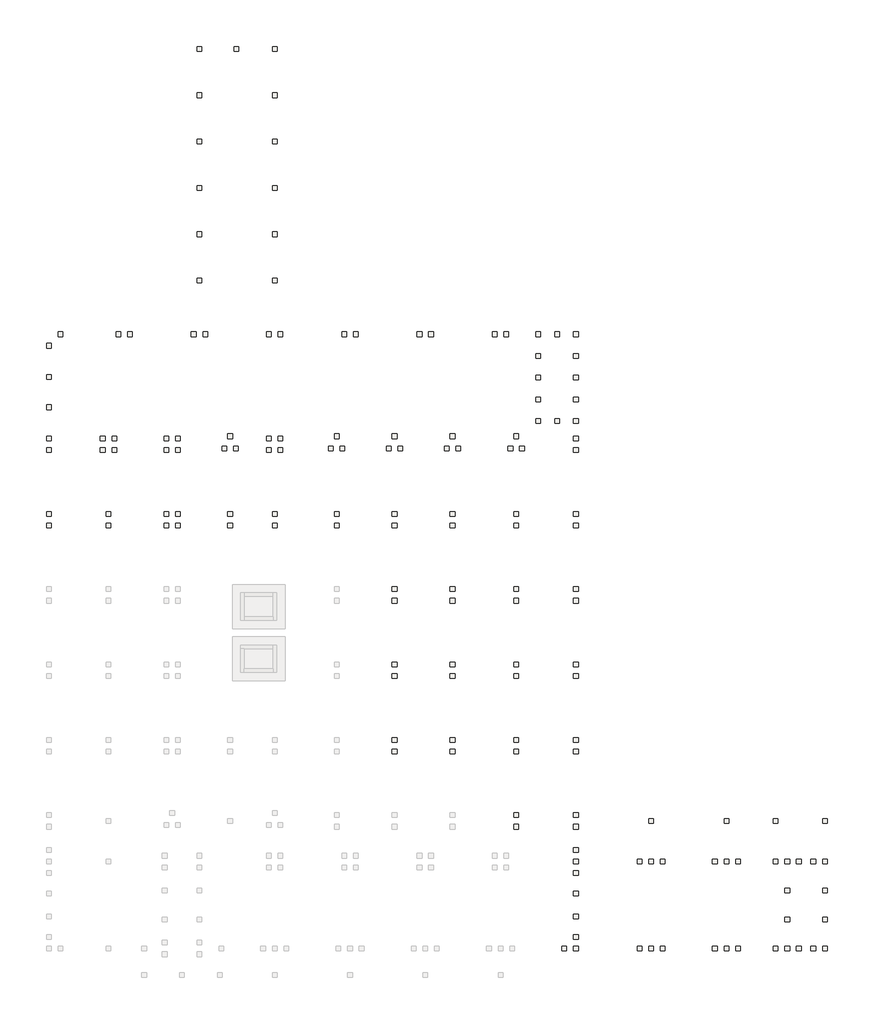
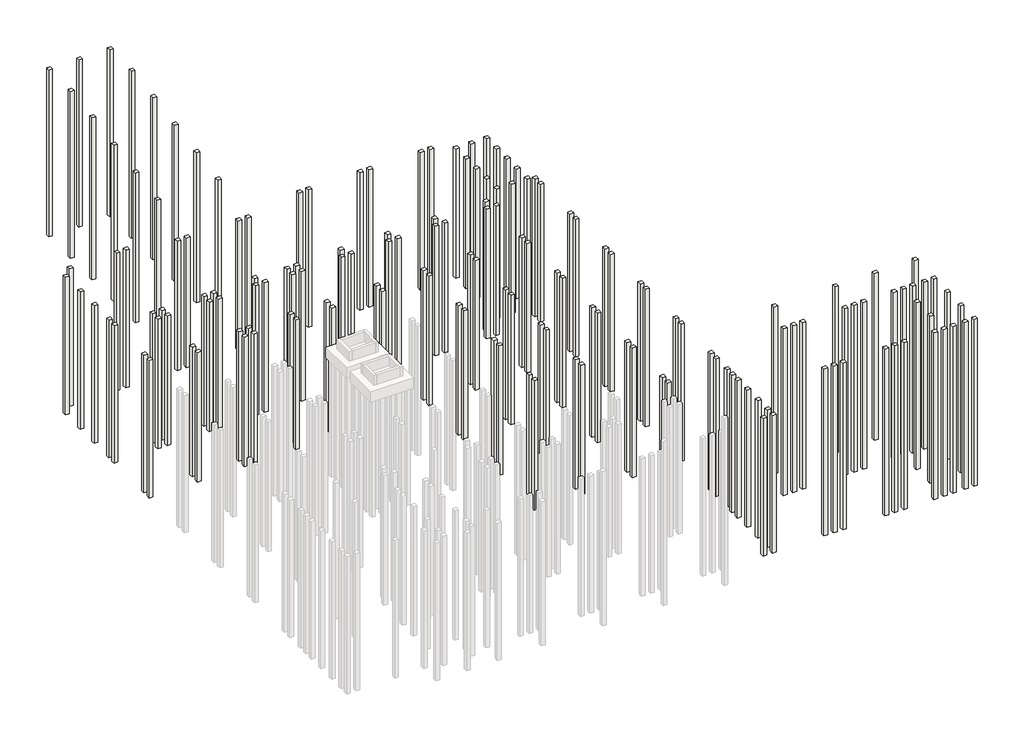
# Not in any storey, part 2 of 2: 160 footings.
# Revit data of these elements (continued)
# Element 105 (IfcFooting, "NLRS_17_SFO_TLB_funderingspaal geheid beton prefab-AV-MMBPC_gen_rsf : heipaal beton prefab_gen__bxh 400x400") (continued)
#   NLRS_S_draagvermogen_druk = 0.00 kN
#   Angle = 0.00°
#   IsExternal = yes
#   LoadBearing = yes
#   Slanted = 0
#   Phase Created = NLRS_nieuw
#   Materials on its faces: "NLRS_f2_beton prefab_gen_rsf"
# Element 106 (IfcFooting, "NLRS_17_SFO_TLB_funderingspaal geheid beton prefab-AV-MMBPC_gen_rsf : heipaal beton prefab_gen__bxh 400x400")
#   IfcGUID = "3loy75XKz2Rw4dS8JWiatC"
#   Slanted Angle = 0.00°
#   NLRS_S_draagvermogen_trek = 0.00 kN
#   NLRS_S_draagvermogen_druk = 0.00 kN
#   Angle = 0.00°
#   IsExternal = yes
#   LoadBearing = yes
#   Slanted = 0
#   Phase Created = NLRS_nieuw
#   Materials on its faces: "NLRS_f2_beton prefab_gen_rsf"
# Element 107 (IfcFooting, "NLRS_17_SFO_TLB_funderingspaal geheid beton prefab-AV-MMBPC_gen_rsf : heipaal beton prefab_gen__bxh 400x400")
#   IfcGUID = "3loy75XKz2Rw4dS8JWiatv"
#   Slanted Angle = 0.00°
#   NLRS_S_draagvermogen_trek = 0.00 kN
#   NLRS_S_draagvermogen_druk = 0.00 kN
#   Angle = 0.00°
#   IsExternal = yes
#   LoadBearing = yes
#   Slanted = 0
#   Phase Created = NLRS_nieuw
#   Materials on its faces: "NLRS_f2_beton prefab_gen_rsf"
# Element 108 (IfcFooting, "NLRS_17_SFO_TLB_funderingspaal geheid beton prefab-AV-MMBPC_gen_rsf : heipaal beton prefab_gen__bxh 400x400")
#   IfcGUID = "3loy75XKz2Rw4dS8JWiat$"
#   Slanted Angle = 0.00°
#   NLRS_S_draagvermogen_trek = 0.00 kN
#   NLRS_S_draagvermogen_druk = 0.00 kN
#   Angle = 0.00°
#   IsExternal = yes
#   LoadBearing = yes
#   Slanted = 0
#   Phase Created = NLRS_nieuw
#   Materials on its faces: "NLRS_f2_beton prefab_gen_rsf"
# Element 109 (IfcFooting, "NLRS_17_SFO_TLB_funderingspaal geheid beton prefab-AV-MMBPC_gen_rsf : heipaal beton prefab_gen__bxh 400x400")
#   IfcGUID = "3loy75XKz2Rw4dS8JWiaEQ"
#   Slanted Angle = 0.00°
#   NLRS_S_draagvermogen_trek = 0.00 kN
#   NLRS_S_draagvermogen_druk = 0.00 kN
#   Angle = 0.00°
#   IsExternal = yes
#   LoadBearing = yes
#   Slanted = 0
#   Phase Created = NLRS_nieuw
#   Materials on its faces: "NLRS_f2_beton prefab_gen_rsf"
# Element 110 (IfcFooting, "NLRS_17_SFO_TLB_funderingspaal geheid beton prefab-AV-MMBPC_gen_rsf : heipaal beton prefab_gen__bxh 400x400")
#   IfcGUID = "3loy75XKz2Rw4dS8JWiaEW"
#   Slanted Angle = 0.00°
#   NLRS_S_draagvermogen_trek = 0.00 kN
#   NLRS_S_draagvermogen_druk = 0.00 kN
#   Angle = 0.00°
#   IsExternal = yes
#   LoadBearing = yes
#   Slanted = 0
#   Phase Created = NLRS_nieuw
#   Materials on its faces: "NLRS_f2_beton prefab_gen_rsf"
# Element 111 (IfcFooting, "NLRS_17_SFO_TLB_funderingspaal geheid beton prefab-AV-MMBPC_gen_rsf : heipaal beton prefab_gen__bxh 400x400")
#   IfcGUID = "3loy75XKz2Rw4dS8JWia10"
#   Slanted Angle = 0.00°
#   NLRS_S_draagvermogen_trek = 0.00 kN
#   NLRS_S_draagvermogen_druk = 0.00 kN
#   Angle = 0.00°
#   IsExternal = yes
#   LoadBearing = yes
#   Slanted = 0
#   Phase Created = NLRS_nieuw
#   Materials on its faces: "NLRS_f2_beton prefab_gen_rsf"
# Element 112 (IfcFooting, "NLRS_17_SFO_TLB_funderingspaal geheid beton prefab-AV-MMBPC_gen_rsf : heipaal beton prefab_gen__bxh 400x400")
#   IfcGUID = "3loy75XKz2Rw4dS8JWia16"
#   Slanted Angle = 0.00°
#   NLRS_S_draagvermogen_trek = 0.00 kN
#   NLRS_S_draagvermogen_druk = 0.00 kN
#   Angle = 0.00°
#   IsExternal = yes
#   LoadBearing = yes
#   Slanted = 0
#   Phase Created = NLRS_nieuw
#   Materials on its faces: "NLRS_f2_beton prefab_gen_rsf"
# Element 113 (IfcFooting, "NLRS_17_SFO_TLB_funderingspaal geheid beton prefab-AV-MMBPC_gen_rsf : heipaal beton prefab_gen__bxh 400x400")
#   IfcGUID = "3loy75XKz2Rw4dS8JWia1p"
#   Slanted Angle = 0.00°
#   NLRS_S_draagvermogen_trek = 0.00 kN
#   NLRS_S_draagvermogen_druk = 0.00 kN
#   Angle = 0.00°
#   IsExternal = yes
#   LoadBearing = yes
#   Slanted = 0
#   Phase Created = NLRS_nieuw
#   Materials on its faces: "NLRS_f2_beton prefab_gen_rsf"
# Element 114 (IfcFooting, "NLRS_17_SFO_TLB_funderingspaal geheid beton prefab-AV-MMBPC_gen_rsf : heipaal beton prefab_gen__bxh 400x400")
#   IfcGUID = "3loy75XKz2Rw4dS8JWia1n"
#   Slanted Angle = 0.00°
#   NLRS_S_draagvermogen_trek = 0.00 kN
#   NLRS_S_draagvermogen_druk = 0.00 kN
#   Angle = 0.00°
#   IsExternal = yes
#   LoadBearing = yes
#   Slanted = 0
#   Phase Created = NLRS_nieuw
#   Materials on its faces: "NLRS_f2_beton prefab_gen_rsf"
# Element 115 (IfcFooting, "NLRS_17_SFO_TLB_funderingspaal geheid beton prefab-AV-MMBPC_gen_rsf : heipaal beton prefab_gen__bxh 400x400")
#   IfcGUID = "3loy75XKz2Rw4dS8JWia5x"
#   Slanted Angle = 0.00°
#   NLRS_S_draagvermogen_trek = 0.00 kN
#   NLRS_S_draagvermogen_druk = 0.00 kN
#   Angle = 0.00°
#   IsExternal = yes
#   LoadBearing = yes
#   Slanted = 0
#   Phase Created = NLRS_nieuw
#   Materials on its faces: "NLRS_f2_beton prefab_gen_rsf"
# Element 116 (IfcFooting, "NLRS_17_SFO_TLB_funderingspaal geheid beton prefab-AV-MMBPC_gen_rsf : heipaal beton prefab_gen__bxh 400x400")
#   IfcGUID = "3loy75XKz2Rw4dS8JWia4Y"
#   Slanted Angle = 0.00°
#   NLRS_S_draagvermogen_trek = 0.00 kN
#   NLRS_S_draagvermogen_druk = 0.00 kN
#   Angle = 0.00°
#   IsExternal = yes
#   LoadBearing = yes
#   Slanted = 0
#   Phase Created = NLRS_nieuw
#   Materials on its faces: "NLRS_f2_beton prefab_gen_rsf"
# Element 117 (IfcFooting, "NLRS_17_SFO_TLB_funderingspaal geheid beton prefab-AV-MMBPC_gen_rsf : heipaal beton prefab_gen__bxh 400x400")
#   IfcGUID = "3loy75XKz2Rw4dS8JWia4W"
#   Slanted Angle = 0.00°
#   NLRS_S_draagvermogen_trek = 0.00 kN
#   NLRS_S_draagvermogen_druk = 0.00 kN
#   Angle = 0.00°
#   IsExternal = yes
#   LoadBearing = yes
#   Slanted = 0
#   Phase Created = NLRS_nieuw
#   Materials on its faces: "NLRS_f2_beton prefab_gen_rsf"
# Element 118 (IfcFooting, "NLRS_17_SFO_TLB_funderingspaal geheid beton prefab-AV-MMBPC_gen_rsf : heipaal beton prefab_gen__bxh 400x400")
#   IfcGUID = "1JrsWFyZX6xPuD52juGVxa"
#   Slanted Angle = 0.00°
#   NLRS_S_draagvermogen_trek = 0.00 kN
#   NLRS_S_draagvermogen_druk = 0.00 kN
#   Angle = 0.00°
#   IsExternal = yes
#   LoadBearing = yes
#   Slanted = 0
#   Phase Created = NLRS_nieuw
#   Materials on its faces: "NLRS_f2_beton prefab_gen_rsf"
# Element 119 (IfcFooting, "NLRS_17_SFO_TLB_funderingspaal geheid beton prefab-AV-MMBPC_gen_rsf : heipaal beton prefab_gen__bxh 400x400")
#   IfcGUID = "1JrsWFyZX6xPuD52juGVvn"
#   Slanted Angle = 0.00°
#   NLRS_S_draagvermogen_trek = 0.00 kN
#   NLRS_S_draagvermogen_druk = 0.00 kN
#   Angle = 0.00°
#   IsExternal = yes
#   LoadBearing = yes
#   Slanted = 0
#   Phase Created = NLRS_nieuw
#   Materials on its faces: "NLRS_f2_beton prefab_gen_rsf"
# Element 120 (IfcFooting, "NLRS_17_SFO_TLB_funderingspaal geheid beton prefab-AV-MMBPC_gen_rsf : heipaal beton prefab_gen__bxh 400x400")
#   IfcGUID = "1JrsWFyZX6xPuD52juGVv2"
#   Slanted Angle = 0.00°
#   NLRS_S_draagvermogen_trek = 0.00 kN
#   NLRS_S_draagvermogen_druk = 0.00 kN
#   Angle = 0.00°
#   IsExternal = yes
#   LoadBearing = yes
#   Slanted = 0
#   Phase Created = NLRS_nieuw
#   Materials on its faces: "NLRS_f2_beton prefab_gen_rsf"
# Element 121 (IfcFooting, "NLRS_17_SFO_TLB_funderingspaal geheid beton prefab-AV-MMBPC_gen_rsf : heipaal beton prefab_gen__bxh 400x400")
#   IfcGUID = "1JrsWFyZX6xPuD52juGV_f"
#   Slanted Angle = 0.00°
#   NLRS_S_draagvermogen_trek = 0.00 kN
#   NLRS_S_draagvermogen_druk = 0.00 kN
#   Angle = 0.00°
#   IsExternal = yes
#   LoadBearing = yes
#   Slanted = 0
#   Phase Created = NLRS_nieuw
#   Materials on its faces: "NLRS_f2_beton prefab_gen_rsf"
# Element 122 (IfcFooting, "NLRS_17_SFO_TLB_funderingspaal geheid beton prefab-AV-MMBPC_gen_rsf : heipaal beton prefab_gen__bxh 400x400")
#   IfcGUID = "1JrsWFyZX6xPuD52juGV_d"
#   Slanted Angle = 0.00°
#   NLRS_S_draagvermogen_trek = 0.00 kN
#   NLRS_S_draagvermogen_druk = 0.00 kN
#   Angle = 0.00°
#   IsExternal = yes
#   LoadBearing = yes
#   Slanted = 0
#   Phase Created = NLRS_nieuw
#   Materials on its faces: "NLRS_f2_beton prefab_gen_rsf"
# Element 123 (IfcFooting, "NLRS_17_SFO_TLB_funderingspaal geheid beton prefab-AV-MMBPC_gen_rsf : heipaal beton prefab_gen__bxh 400x400")
#   IfcGUID = "1JrsWFyZX6xPuD52juGV_b"
#   Slanted Angle = 0.00°
#   NLRS_S_draagvermogen_trek = 0.00 kN
#   NLRS_S_draagvermogen_druk = 0.00 kN
#   Angle = 0.00°
#   IsExternal = yes
#   LoadBearing = yes
#   Slanted = 0
#   Phase Created = NLRS_nieuw
#   Materials on its faces: "NLRS_f2_beton prefab_gen_rsf"
# Element 124 (IfcFooting, "NLRS_17_SFO_TLB_funderingspaal geheid beton prefab-AV-MMBPC_gen_rsf : heipaal beton prefab_gen__bxh 400x400")
#   IfcGUID = "1JrsWFyZX6xPuD52juGV_G"
#   Slanted Angle = 0.00°
#   NLRS_S_draagvermogen_trek = 0.00 kN
#   NLRS_S_draagvermogen_druk = 0.00 kN
#   Angle = 0.00°
#   IsExternal = yes
#   LoadBearing = yes
#   Slanted = 0
#   Phase Created = NLRS_nieuw
#   Materials on its faces: "NLRS_f2_beton prefab_gen_rsf"
# Element 125 (IfcFooting, "NLRS_17_SFO_TLB_funderingspaal geheid beton prefab-AV-MMBPC_gen_rsf : heipaal beton prefab_gen__bxh 400x400")
#   IfcGUID = "1JrsWFyZX6xPuD52juGV_E"
#   Slanted Angle = 0.00°
#   NLRS_S_draagvermogen_trek = 0.00 kN
#   NLRS_S_draagvermogen_druk = 0.00 kN
#   Angle = 0.00°
#   IsExternal = yes
#   LoadBearing = yes
#   Slanted = 0
#   Phase Created = NLRS_nieuw
#   Materials on its faces: "NLRS_f2_beton prefab_gen_rsf"
# Element 126 (IfcFooting, "NLRS_17_SFO_TLB_funderingspaal geheid beton prefab-AV-MMBPC_gen_rsf : heipaal beton prefab_gen__bxh 400x400")
#   IfcGUID = "1JrsWFyZX6xPuD52juGV_C"
#   Slanted Angle = 0.00°
#   NLRS_S_draagvermogen_trek = 0.00 kN
#   NLRS_S_draagvermogen_druk = 0.00 kN
#   Angle = 0.00°
#   IsExternal = yes
#   LoadBearing = yes
#   Slanted = 0
#   Phase Created = NLRS_nieuw
#   Materials on its faces: "NLRS_f2_beton prefab_gen_rsf"
# Element 127 (IfcFooting, "NLRS_17_SFO_TLB_funderingspaal geheid beton prefab-AV-MMBPC_gen_rsf : heipaal beton prefab_gen__bxh 400x400")
#   IfcGUID = "1JrsWFyZX6xPuD52juGV_A"
#   Slanted Angle = 0.00°
#   NLRS_S_draagvermogen_trek = 0.00 kN
#   NLRS_S_draagvermogen_druk = 0.00 kN
#   Angle = 0.00°
#   IsExternal = yes
#   LoadBearing = yes
#   Slanted = 0
#   Phase Created = NLRS_nieuw
#   Materials on its faces: "NLRS_f2_beton prefab_gen_rsf"
# Element 128 (IfcFooting, "NLRS_17_SFO_TLB_funderingspaal geheid beton prefab-AV-MMBPC_gen_rsf : heipaal beton prefab_gen__bxh 400x400")
#   IfcGUID = "1JrsWFyZX6xPuD52juGV_8"
#   Slanted Angle = 0.00°
#   NLRS_S_draagvermogen_trek = 0.00 kN
#   NLRS_S_draagvermogen_druk = 0.00 kN
#   Angle = 0.00°
#   IsExternal = yes
#   LoadBearing = yes
#   Slanted = 0
#   Phase Created = NLRS_nieuw
#   Materials on its faces: "NLRS_f2_beton prefab_gen_rsf"
# Element 129 (IfcFooting, "NLRS_17_SFO_TLB_funderingspaal geheid beton prefab-AV-MMBPC_gen_rsf : heipaal beton prefab_gen__bxh 400x400")
#   IfcGUID = "1JrsWFyZX6xPuD52juGV_6"
#   Slanted Angle = 0.00°
#   NLRS_S_draagvermogen_trek = 0.00 kN
#   NLRS_S_draagvermogen_druk = 0.00 kN
#   Angle = 0.00°
#   IsExternal = yes
#   LoadBearing = yes
#   Slanted = 0
#   Phase Created = NLRS_nieuw
#   Materials on its faces: "NLRS_f2_beton prefab_gen_rsf"
# Element 130 (IfcFooting, "NLRS_17_SFO_TLB_funderingspaal geheid beton prefab-AV-MMBPC_gen_rsf : heipaal beton prefab_gen__bxh 400x400")
#   IfcGUID = "1JrsWFyZX6xPuD52juGV$T"
#   Slanted Angle = 0.00°
#   NLRS_S_draagvermogen_trek = 0.00 kN
#   NLRS_S_draagvermogen_druk = 0.00 kN
#   Angle = 0.00°
#   IsExternal = yes
#   LoadBearing = yes
#   Slanted = 0
#   Phase Created = NLRS_nieuw
#   Materials on its faces: "NLRS_f2_beton prefab_gen_rsf"
# Element 131 (IfcFooting, "NLRS_17_SFO_TLB_funderingspaal geheid beton prefab-AV-MMBPC_gen_rsf : heipaal beton prefab_gen__bxh 400x400")
#   IfcGUID = "1JrsWFyZX6xPuD52juGV$G"
#   Slanted Angle = 0.00°
#   NLRS_S_draagvermogen_trek = 0.00 kN
#   NLRS_S_draagvermogen_druk = 0.00 kN
#   Angle = 0.00°
#   IsExternal = yes
#   LoadBearing = yes
#   Slanted = 0
#   Phase Created = NLRS_nieuw
#   Materials on its faces: "NLRS_f2_beton prefab_gen_rsf"
# Element 132 (IfcFooting, "NLRS_17_SFO_TLB_funderingspaal geheid beton prefab-AV-MMBPC_gen_rsf : heipaal beton prefab_gen__bxh 400x400")
#   IfcGUID = "1JrsWFyZX6xPuD52juGVyj"
#   Slanted Angle = 0.00°
#   NLRS_S_draagvermogen_trek = 0.00 kN
#   NLRS_S_draagvermogen_druk = 0.00 kN
#   Angle = 0.00°
#   IsExternal = yes
#   LoadBearing = yes
#   Slanted = 0
#   Phase Created = NLRS_nieuw
#   Materials on its faces: "NLRS_f2_beton prefab_gen_rsf"
# Element 133 (IfcFooting, "NLRS_17_SFO_TLB_funderingspaal geheid beton prefab-AV-MMBPC_gen_rsf : heipaal beton prefab_gen__bxh 400x400")
#   IfcGUID = "1JrsWFyZX6xPuD52juGVy1"
#   Slanted Angle = 0.00°
#   NLRS_S_draagvermogen_trek = 0.00 kN
#   NLRS_S_draagvermogen_druk = 0.00 kN
#   Angle = 0.00°
#   IsExternal = yes
#   LoadBearing = yes
#   Slanted = 0
#   Phase Created = NLRS_nieuw
#   Materials on its faces: "NLRS_f2_beton prefab_gen_rsf"
# Element 134 (IfcFooting, "NLRS_17_SFO_TLB_funderingspaal geheid beton prefab-AV-MMBPC_gen_rsf : heipaal beton prefab_gen__bxh 400x400")
#   IfcGUID = "1JrsWFyZX6xPuD52juGVz$"
#   Slanted Angle = 0.00°
#   NLRS_S_draagvermogen_trek = 0.00 kN
#   NLRS_S_draagvermogen_druk = 0.00 kN
#   Angle = 0.00°
#   IsExternal = yes
#   LoadBearing = yes
#   Slanted = 0
#   Phase Created = NLRS_nieuw
#   Materials on its faces: "NLRS_f2_beton prefab_gen_rsf"
# Element 135 (IfcFooting, "NLRS_17_SFO_TLB_funderingspaal geheid beton prefab-AV-MMBPC_gen_rsf : heipaal beton prefab_gen__bxh 400x400")
#   IfcGUID = "1JrsWFyZX6xPuD52juGVzz"
#   Slanted Angle = 0.00°
#   NLRS_S_draagvermogen_trek = 0.00 kN
#   NLRS_S_draagvermogen_druk = 0.00 kN
#   Angle = 0.00°
#   IsExternal = yes
#   LoadBearing = yes
#   Slanted = 0
#   Phase Created = NLRS_nieuw
#   Materials on its faces: "NLRS_f2_beton prefab_gen_rsf"
# Element 136 (IfcFooting, "NLRS_17_SFO_TLB_funderingspaal geheid beton prefab-AV-MMBPC_gen_rsf : heipaal beton prefab_gen__bxh 400x400")
#   IfcGUID = "1JrsWFyZX6xPuD52juGVzI"
#   Slanted Angle = 0.00°
#   NLRS_S_draagvermogen_trek = 0.00 kN
#   NLRS_S_draagvermogen_druk = 0.00 kN
#   Angle = 0.00°
#   IsExternal = yes
#   LoadBearing = yes
#   Slanted = 0
#   Phase Created = NLRS_nieuw
#   Materials on its faces: "NLRS_f2_beton prefab_gen_rsf"
# Element 137 (IfcFooting, "NLRS_17_SFO_TLB_funderingspaal geheid beton prefab-AV-MMBPC_gen_rsf : heipaal beton prefab_gen__bxh 400x400")
#   IfcGUID = "1JrsWFyZX6xPuD52juGVz7"
#   Slanted Angle = 0.00°
#   NLRS_S_draagvermogen_trek = 0.00 kN
#   NLRS_S_draagvermogen_druk = 0.00 kN
#   Angle = 0.00°
#   IsExternal = yes
#   LoadBearing = yes
#   Slanted = 0
#   Phase Created = NLRS_nieuw
#   Materials on its faces: "NLRS_f2_beton prefab_gen_rsf"
# Element 138 (IfcFooting, "NLRS_17_SFO_TLB_funderingspaal geheid beton prefab-AV-MMBPC_gen_rsf : heipaal beton prefab_gen__bxh 400x400")
#   IfcGUID = "1JrsWFyZX6xPuD52juGVog"
#   Slanted Angle = 0.00°
#   NLRS_S_draagvermogen_trek = 0.00 kN
#   NLRS_S_draagvermogen_druk = 0.00 kN
#   Angle = 0.00°
#   IsExternal = yes
#   LoadBearing = yes
#   Slanted = 0
#   Phase Created = NLRS_nieuw
#   Materials on its faces: "NLRS_f2_beton prefab_gen_rsf"
# Element 139 (IfcFooting, "NLRS_17_SFO_TLB_funderingspaal geheid beton prefab-AV-MMBPC_gen_rsf : heipaal beton prefab_gen__bxh 400x400")
#   IfcGUID = "1JrsWFyZX6xPuD52juGVoe"
#   Slanted Angle = 0.00°
#   NLRS_S_draagvermogen_trek = 0.00 kN
#   NLRS_S_draagvermogen_druk = 0.00 kN
#   Angle = 0.00°
#   IsExternal = yes
#   LoadBearing = yes
#   Slanted = 0
#   Phase Created = NLRS_nieuw
#   Materials on its faces: "NLRS_f2_beton prefab_gen_rsf"
# Element 140 (IfcFooting, "NLRS_17_SFO_TLB_funderingspaal geheid beton prefab-AV-MMBPC_gen_rsf : heipaal beton prefab_gen__bxh 400x400")
#   IfcGUID = "1JrsWFyZX6xPuD52juGVpj"
#   Slanted Angle = 0.00°
#   NLRS_S_draagvermogen_trek = 0.00 kN
#   NLRS_S_draagvermogen_druk = 0.00 kN
#   Angle = 0.00°
#   IsExternal = yes
#   LoadBearing = yes
#   Slanted = 0
#   Phase Created = NLRS_nieuw
#   Materials on its faces: "NLRS_f2_beton prefab_gen_rsf"
# Element 141 (IfcFooting, "NLRS_17_SFO_TLB_funderingspaal geheid beton prefab-AV-MMBPC_gen_rsf : heipaal beton prefab_gen__bxh 400x400")
#   IfcGUID = "1JrsWFyZX6xPuD52juGVph"
#   Slanted Angle = 0.00°
#   NLRS_S_draagvermogen_trek = 0.00 kN
#   NLRS_S_draagvermogen_druk = 0.00 kN
#   Angle = 0.00°
#   IsExternal = yes
#   LoadBearing = yes
#   Slanted = 0
#   Phase Created = NLRS_nieuw
#   Materials on its faces: "NLRS_f2_beton prefab_gen_rsf"
# Element 142 (IfcFooting, "NLRS_17_SFO_TLB_funderingspaal geheid beton prefab-AV-MMBPC_gen_rsf : heipaal beton prefab_gen__bxh 400x400")
#   IfcGUID = "1JrsWFyZX6xPuD52juGVp8"
#   Slanted Angle = 0.00°
#   NLRS_S_draagvermogen_trek = 0.00 kN
#   NLRS_S_draagvermogen_druk = 0.00 kN
#   Angle = 0.00°
#   IsExternal = yes
#   LoadBearing = yes
#   Slanted = 0
#   Phase Created = NLRS_nieuw
#   Materials on its faces: "NLRS_f2_beton prefab_gen_rsf"
# Element 143 (IfcFooting, "NLRS_17_SFO_TLB_funderingspaal geheid beton prefab-AV-MMBPC_gen_rsf : heipaal beton prefab_gen__bxh 400x400")
#   IfcGUID = "1JrsWFyZX6xPuD52juGVp6"
#   Slanted Angle = 0.00°
#   NLRS_S_draagvermogen_trek = 0.00 kN
#   NLRS_S_draagvermogen_druk = 0.00 kN
#   Angle = 0.00°
#   IsExternal = yes
#   LoadBearing = yes
#   Slanted = 0
#   Phase Created = NLRS_nieuw
#   Materials on its faces: "NLRS_f2_beton prefab_gen_rsf"
# Element 144 (IfcFooting, "NLRS_17_SFO_TLB_funderingspaal geheid beton prefab-AV-MMBPC_gen_rsf : heipaal beton prefab_gen__bxh 400x400")
#   IfcGUID = "1JrsWFyZX6xPuD52juGVmn"
#   Slanted Angle = 0.00°
#   NLRS_S_draagvermogen_trek = 0.00 kN
#   NLRS_S_draagvermogen_druk = 0.00 kN
#   Angle = 0.00°
#   IsExternal = yes
#   LoadBearing = yes
#   Slanted = 0
#   Phase Created = NLRS_nieuw
#   Materials on its faces: "NLRS_f2_beton prefab_gen_rsf"
# Element 145 (IfcFooting, "NLRS_17_SFO_TLB_funderingspaal geheid beton prefab-AV-MMBPC_gen_rsf : heipaal beton prefab_gen__bxh 400x400")
#   IfcGUID = "1JrsWFyZX6xPuD52juGVm6"
#   Slanted Angle = 0.00°
#   NLRS_S_draagvermogen_trek = 0.00 kN
#   NLRS_S_draagvermogen_druk = 0.00 kN
#   Angle = 0.00°
#   IsExternal = yes
#   LoadBearing = yes
#   Slanted = 0
#   Phase Created = NLRS_nieuw
#   Materials on its faces: "NLRS_f2_beton prefab_gen_rsf"
# Element 146 (IfcFooting, "NLRS_17_SFO_TLB_funderingspaal geheid beton prefab-AV-MMBPC_gen_rsf : heipaal beton prefab_gen__bxh 400x400")
#   IfcGUID = "1JrsWFyZX6xPuD52juGVnx"
#   Slanted Angle = 0.00°
#   NLRS_S_draagvermogen_trek = 0.00 kN
#   NLRS_S_draagvermogen_druk = 0.00 kN
#   Angle = 0.00°
#   IsExternal = yes
#   LoadBearing = yes
#   Slanted = 0
#   Phase Created = NLRS_nieuw
#   Materials on its faces: "NLRS_f2_beton prefab_gen_rsf"
# Element 147 (IfcFooting, "NLRS_17_SFO_TLB_funderingspaal geheid beton prefab-AV-MMBPC_gen_rsf : heipaal beton prefab_gen__bxh 400x400")
#   IfcGUID = "1JrsWFyZX6xPuD52juGVnv"
#   Slanted Angle = 0.00°
#   NLRS_S_draagvermogen_trek = 0.00 kN
#   NLRS_S_draagvermogen_druk = 0.00 kN
#   Angle = 0.00°
#   IsExternal = yes
#   LoadBearing = yes
#   Slanted = 0
#   Phase Created = NLRS_nieuw
#   Materials on its faces: "NLRS_f2_beton prefab_gen_rsf"
# Element 148 (IfcFooting, "NLRS_17_SFO_TLB_funderingspaal geheid beton prefab-AV-MMBPC_gen_rsf : heipaal beton prefab_gen__bxh 400x400")
#   IfcGUID = "3aMdMHoe12P9KDGPyaIhq7"
#   Slanted Angle = 0.00°
#   NLRS_S_draagvermogen_trek = 0.00 kN
#   NLRS_S_draagvermogen_druk = 0.00 kN
#   Angle = 0.00°
#   IsExternal = yes
#   LoadBearing = yes
#   Slanted = 0
#   Phase Created = NLRS_nieuw
#   Materials on its faces: "NLRS_f2_beton prefab_gen_rsf"
# Element 149 (IfcFooting, "NLRS_17_SFO_TLB_funderingspaal geheid beton prefab-AV-MMBPC_gen_rsf : heipaal beton prefab_gen__bxh 400x400")
#   IfcGUID = "3aMdMHoe12P9KDGPyaIhqK"
#   Slanted Angle = 0.00°
#   NLRS_S_draagvermogen_trek = 0.00 kN
#   NLRS_S_draagvermogen_druk = 0.00 kN
#   Angle = 0.00°
#   IsExternal = yes
#   LoadBearing = yes
#   Slanted = 0
#   Phase Created = NLRS_nieuw
#   Materials on its faces: "NLRS_f2_beton prefab_gen_rsf"
# Element 150 (IfcFooting, "NLRS_17_SFO_TLB_funderingspaal geheid beton prefab-AV-MMBPC_gen_rsf : heipaal beton prefab_gen__bxh 400x400")
#   IfcGUID = "3aMdMHoe12P9KDGPyaIhth"
#   Slanted Angle = 0.00°
#   NLRS_S_draagvermogen_trek = 0.00 kN
#   NLRS_S_draagvermogen_druk = 0.00 kN
#   Angle = 0.00°
#   IsExternal = yes
#   LoadBearing = yes
#   Slanted = 0
#   Phase Created = NLRS_nieuw
#   Materials on its faces: "NLRS_f2_beton prefab_gen_rsf"
# Element 151 (IfcFooting, "NLRS_17_SFO_TLB_funderingspaal geheid beton prefab-AV-MMBPC_gen_rsf : heipaal beton prefab_gen__bxh 400x400")
#   IfcGUID = "3aMdMHoe12P9KDGPyaIht6"
#   Slanted Angle = 0.00°
#   NLRS_S_draagvermogen_trek = 0.00 kN
#   NLRS_S_draagvermogen_druk = 0.00 kN
#   Angle = 0.00°
#   IsExternal = yes
#   LoadBearing = yes
#   Slanted = 0
#   Phase Created = NLRS_nieuw
#   Materials on its faces: "NLRS_f2_beton prefab_gen_rsf"
# Element 152 (IfcFooting, "NLRS_17_SFO_TLB_funderingspaal geheid beton prefab-AV-MMBPC_gen_rsf : heipaal beton prefab_gen__bxh 400x400")
#   IfcGUID = "3aMdMHoe12P9KDGPyaIhtP"
#   Slanted Angle = 0.00°
#   NLRS_S_draagvermogen_trek = 0.00 kN
#   NLRS_S_draagvermogen_druk = 0.00 kN
#   Angle = 0.00°
#   IsExternal = yes
#   LoadBearing = yes
#   Slanted = 0
#   Phase Created = NLRS_nieuw
#   Materials on its faces: "NLRS_f2_beton prefab_gen_rsf"
# Element 153 (IfcFooting, "NLRS_17_SFO_TLB_funderingspaal geheid beton prefab-AV-MMBPC_gen_rsf : heipaal beton prefab_gen__bxh 400x400")
#   IfcGUID = "3aMdMHoe12P9KDGPyaIhsw"
#   Slanted Angle = 0.00°
#   NLRS_S_draagvermogen_trek = 0.00 kN
#   NLRS_S_draagvermogen_druk = 0.00 kN
#   Angle = 0.00°
#   IsExternal = yes
#   LoadBearing = yes
#   Slanted = 0
#   Phase Created = NLRS_nieuw
#   Materials on its faces: "NLRS_f2_beton prefab_gen_rsf"
# Element 154 (IfcFooting, "NLRS_17_SFO_TLB_funderingspaal geheid beton prefab-AV-MMBPC_gen_rsf : heipaal beton prefab_gen__bxh 400x400")
#   IfcGUID = "3aMdMHoe12P9KDGPyaIhxf"
#   Slanted Angle = 0.00°
#   NLRS_S_draagvermogen_trek = 0.00 kN
#   NLRS_S_draagvermogen_druk = 0.00 kN
#   Angle = 0.00°
#   IsExternal = yes
#   LoadBearing = yes
#   Slanted = 0
#   Phase Created = NLRS_nieuw
#   Materials on its faces: "NLRS_f2_beton prefab_gen_rsf"
# Element 155 (IfcFooting, "NLRS_17_SFO_TLB_funderingspaal geheid beton prefab-AV-MMBPC_gen_rsf : heipaal beton prefab_gen__bxh 400x400")
#   IfcGUID = "3aMdMHoe12P9KDGPyaIhsp"
#   Slanted Angle = 0.00°
#   NLRS_S_draagvermogen_trek = 0.00 kN
#   NLRS_S_draagvermogen_druk = 0.00 kN
#   Angle = 0.00°
#   IsExternal = yes
#   LoadBearing = yes
#   Slanted = 0
#   Phase Created = NLRS_nieuw
#   Materials on its faces: "NLRS_f2_beton prefab_gen_rsf"
# Element 156 (IfcFooting, "NLRS_17_SFO_TLB_funderingspaal geheid beton prefab-AV-MMBPC_gen_rsf : heipaal beton prefab_gen__bxh 400x400")
#   IfcGUID = "3aMdMHoe12P9KDGPyaIhxd"
#   Slanted Angle = 0.00°
#   NLRS_S_draagvermogen_trek = 0.00 kN
#   NLRS_S_draagvermogen_druk = 0.00 kN
#   Angle = 0.00°
#   IsExternal = yes
#   LoadBearing = yes
#   Slanted = 0
#   Phase Created = NLRS_nieuw
#   Materials on its faces: "NLRS_f2_beton prefab_gen_rsf"
# Element 157 (IfcFooting, "NLRS_17_SFO_TLB_funderingspaal geheid beton prefab-AV-MMBPC_gen_rsf : heipaal beton prefab_gen__bxh 400x400")
#   IfcGUID = "3aMdMHoe12P9KDGPyaIhs8"
#   Slanted Angle = 0.00°
#   NLRS_S_draagvermogen_trek = 0.00 kN
#   NLRS_S_draagvermogen_druk = 0.00 kN
#   Angle = 0.00°
#   IsExternal = yes
#   LoadBearing = yes
#   Slanted = 0
#   Phase Created = NLRS_nieuw
#   Materials on its faces: "NLRS_f2_beton prefab_gen_rsf"
# Element 158 (IfcFooting, "NLRS_17_SFO_TLB_funderingspaal geheid beton prefab-AV-MMBPC_gen_rsf : heipaal beton prefab_gen__bxh 400x400")
#   IfcGUID = "3aMdMHoe12P9KDGPyaIhxb"
#   Slanted Angle = 0.00°
#   NLRS_S_draagvermogen_trek = 0.00 kN
#   NLRS_S_draagvermogen_druk = 0.00 kN
#   Angle = 0.00°
#   IsExternal = yes
#   LoadBearing = yes
#   Slanted = 0
#   Phase Created = NLRS_nieuw
#   Materials on its faces: "NLRS_f2_beton prefab_gen_rsf"
# Element 159 (IfcFooting, "NLRS_17_SFO_TLB_funderingspaal geheid beton prefab-AV-MMBPC_gen_rsf : heipaal beton prefab_gen__bxh 400x400")
#   IfcGUID = "3aMdMHoe12P9KDGPyaIhs1"
#   Slanted Angle = 0.00°
#   NLRS_S_draagvermogen_trek = 0.00 kN
#   NLRS_S_draagvermogen_druk = 0.00 kN
#   Angle = 0.00°
#   IsExternal = yes
#   LoadBearing = yes
#   Slanted = 0
#   Phase Created = NLRS_nieuw
#   Materials on its faces: "NLRS_f2_beton prefab_gen_rsf"
# Element 160 (IfcFooting, "NLRS_17_SFO_TLB_funderingspaal geheid beton prefab-AV-MMBPC_gen_rsf : heipaal beton prefab_gen__bxh 400x400")
#   IfcGUID = "3aMdMHoe12P9KDGPyaIhxZ"
#   Slanted Angle = 0.00°
#   NLRS_S_draagvermogen_trek = 0.00 kN
#   NLRS_S_draagvermogen_druk = 0.00 kN
#   Angle = 0.00°
#   IsExternal = yes
#   LoadBearing = yes
#   Slanted = 0
#   Phase Created = NLRS_nieuw
#   Materials on its faces: "NLRS_f2_beton prefab_gen_rsf"
# Materials
#   "NLRS_f2_beton prefab_gen_rsf": class "F - Niet gebakken kunststeen", colour RGB 129 133 118, transparency 0, Keynote = "f2", Manufacturer = "Revit Standards Foundation", URL = "www.revitstandards.org", Description = "beton prefab", Cost = 0
